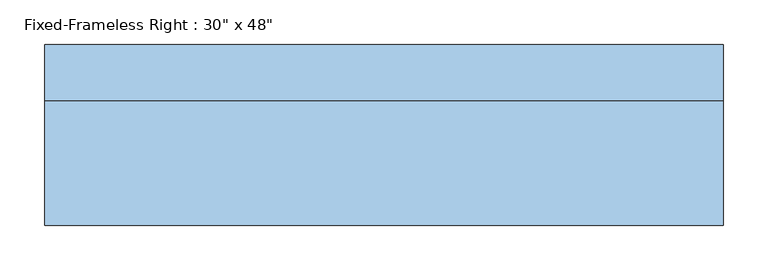
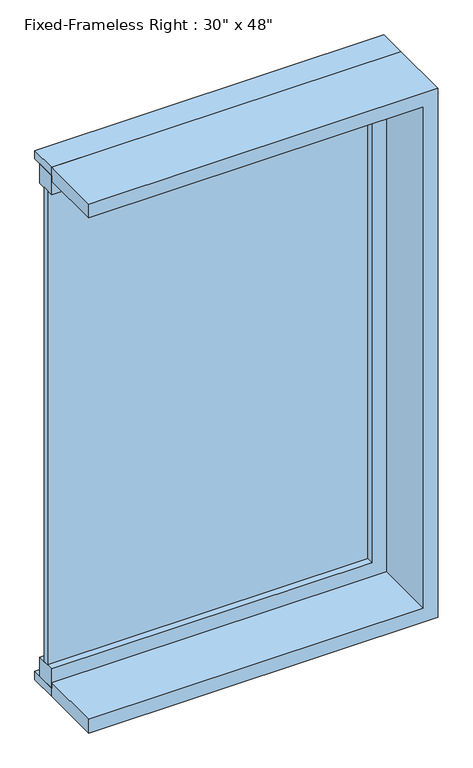
"""IFC4 building model written with IfcOpenShell, lengths in millimetres: window geometry."""

import ifcopenshell
import ifcopenshell.guid

model = None  # the IFC model being written
_history = None  # IfcOwnerHistory: only IFC2X3 demands one
_inside = {}  # id of a spatial element -> (the spatial element, [elements in it])
_under = {}  # id of a project, library or spatial element -> (it, [spatial elements below it])
_declared = {}  # id of a project -> (the project, [libraries it declares])
_typed = {}  # id of a type object -> (the type object, [elements of that type])
_made_of = {}  # id of a material, layer set ... -> (it, [elements and type objects made of it])


def new_model(schema):
    """Start an empty IFC model of exactly this schema.

    Asked for "IFC4X3", IfcOpenShell would pick the latest addendum, in which some entities
    have other attributes; the version numbers below select the first issue.
    IFC2X3 requires an IfcOwnerHistory on every rooted entity: one is made here for all.
    """
    global model, _history
    if schema == "IFC4X3":
        model = ifcopenshell.file(schema_version=(4, 3, 0, 0))
    else:
        model = ifcopenshell.file(schema=schema)
    _inside.clear()
    _under.clear()
    _declared.clear()
    _typed.clear()
    _made_of.clear()
    _history = None
    if model.schema == "IFC2X3":
        org = make("IfcOrganization", Name="unknown")
        user = make(
            "IfcPersonAndOrganization",
            ThePerson=make("IfcPerson", FamilyName="unknown"),
            TheOrganization=org,
        )
        app = make(
            "IfcApplication",
            ApplicationDeveloper=org,
            Version="unknown",
            ApplicationFullName="unknown",
            ApplicationIdentifier="unknown",
        )
        _history = make(
            "IfcOwnerHistory",
            OwningUser=user,
            OwningApplication=app,
            ChangeAction="ADDED",
            CreationDate=0,
        )
    return model


def make(cls, **values):
    """One entity of the class cls with the attributes given. An attribute that is None is left unset."""
    return model.create_entity(
        cls, **{name: value for name, value in values.items() if value is not None}
    )


def rooted(cls, **values):
    """An entity with a GlobalId (a new one), such as an element, a storey or a relation."""
    return make(cls, GlobalId=ifcopenshell.guid.new(), OwnerHistory=_history, **values)


def si_unit(unit_type, name, prefix=None):
    """IfcSIUnit, for example si_unit("LENGTHUNIT", "METRE", prefix="MILLI")."""
    return make("IfcSIUnit", UnitType=unit_type, Prefix=prefix, Name=name)


def assignment(units):
    """IfcUnitAssignment: the units of a project."""
    return None if units is None else make("IfcUnitAssignment", Units=units)


def point(xyz):
    """IfcCartesianPoint."""
    return None if xyz is None else make("IfcCartesianPoint", Coordinates=xyz)


def direction(xyz):
    """IfcDirection."""
    return None if xyz is None else make("IfcDirection", DirectionRatios=xyz)


def frame(location, z_axis=None, x_axis=None):
    """IfcAxis2Placement3D, a coordinate frame: its origin and axes. An axis left out is left unset."""
    return make(
        "IfcAxis2Placement3D",
        Location=point(location),
        Axis=direction(z_axis),
        RefDirection=direction(x_axis),
    )


def origin():
    """The frame at (0, 0, 0) with its axes left unset."""
    return frame((0.0, 0.0, 0.0))


def place(relative_to, where):
    """IfcLocalPlacement: puts the frame where relative to a parent placement (None: the world)."""
    return make(
        "IfcLocalPlacement", PlacementRelTo=relative_to, RelativePlacement=where
    )


def context(
    kind, dimensions, precision=None, world=None, true_north=None, identifier=None
):
    """IfcGeometricRepresentationContext, for example the 3D "Model" context."""
    return make(
        "IfcGeometricRepresentationContext",
        ContextIdentifier=identifier,
        ContextType=kind,
        CoordinateSpaceDimension=dimensions,
        Precision=precision,
        WorldCoordinateSystem=world,
        TrueNorth=true_north,
    )


def project(units=None, contexts=None):
    """IfcProject with its units and contexts."""
    return rooted(
        "IfcProject",
        Name="project",
        RepresentationContexts=contexts,
        UnitsInContext=assignment(units),
    )


def spatial(cls, under=None, at=None, **own):
    """A site, building, storey or space (cls), placed at a placement, below another one or the project."""
    s = rooted(cls, ObjectPlacement=at, **own)
    if under is not None:
        _under.setdefault(under.id(), (under, []))[1].append(s)
    return s


def polyline(points):
    """IfcPolyline through the points."""
    return make("IfcPolyline", Points=[point(p) for p in points])


def outline(outer, holes=None, kind="AREA"):
    """IfcArbitraryClosedProfileDef: a profile drawn as a closed curve; with holes, ...WithVoids."""
    if holes is None:
        return make("IfcArbitraryClosedProfileDef", ProfileType=kind, OuterCurve=outer)
    return make(
        "IfcArbitraryProfileDefWithVoids",
        ProfileType=kind,
        OuterCurve=outer,
        InnerCurves=holes,
    )


def extrude(swept, where, along, depth):
    """IfcExtrudedAreaSolid: the profile swept, set in the frame where, extruded along a direction by depth."""
    return make(
        "IfcExtrudedAreaSolid",
        SweptArea=swept,
        Position=where,
        ExtrudedDirection=direction(along),
        Depth=depth,
    )


def shape(context_of_items, identifier, shape_type, items):
    """IfcShapeRepresentation: the items that make up one representation, for example the "Body"."""
    return make(
        "IfcShapeRepresentation",
        ContextOfItems=context_of_items,
        RepresentationIdentifier=identifier,
        RepresentationType=shape_type,
        Items=items,
    )


def source(mapping_origin, context_of_items, identifier, shape_type, items):
    """IfcRepresentationMap: a shape defined once, which mapped items show again and again."""
    return make(
        "IfcRepresentationMap",
        MappingOrigin=mapping_origin,
        MappedRepresentation=shape(context_of_items, identifier, shape_type, items),
    )


def transform(
    local_origin,
    x_axis=None,
    y_axis=None,
    z_axis=None,
    scale=None,
    scale2=None,
    scale3=None,
    uniform=True,
):
    """IfcCartesianTransformationOperator3D, or its non-uniform kind. x_axis, y_axis, z_axis: its Axis1, 2, 3."""
    if uniform:
        return make(
            "IfcCartesianTransformationOperator3D",
            Axis1=direction(x_axis),
            Axis2=direction(y_axis),
            LocalOrigin=point(local_origin),
            Scale=scale,
            Axis3=direction(z_axis),
        )
    return make(
        "IfcCartesianTransformationOperator3DnonUniform",
        Axis1=direction(x_axis),
        Axis2=direction(y_axis),
        LocalOrigin=point(local_origin),
        Scale=scale,
        Axis3=direction(z_axis),
        Scale2=scale2,
        Scale3=scale3,
    )


def mapped(mapping_source, mapping_target):
    """IfcMappedItem: shows the shape of a source again, moved by a transform."""
    return make(
        "IfcMappedItem", MappingSource=mapping_source, MappingTarget=mapping_target
    )


def made_of(thing, what):
    """Note that an element or type object is made of a material, layer set ...; save() writes the relation."""
    if what is not None:
        _made_of.setdefault(what.id(), (what, []))[1].append(thing)
    return thing


def element(
    cls,
    number,
    at=None,
    inside=None,
    cuts=None,
    type_object=None,
    material=None,
    context=None,
    identifier="Body",
    shape_type=None,
    held_by="IfcProductDefinitionShape",
    body=None,
    shapes=None,
    **own,
):
    """One element of the class cls, such as IfcWall. Its Tag is "e" and its number.

    at: its placement. inside: the storey or other place that contains it. cuts: it is an
    opening in that element (IfcRelVoidsElement). A single representation is given by context,
    identifier, shape_type and body (its items); several are given by shapes. held_by: the class
    of the entity that holds the representations. save() writes the other relations.
    """
    e = rooted(cls, Tag="e%d" % number, ObjectPlacement=at, **own)
    if body is not None:
        shapes = [shape(context, identifier, shape_type, body)]
    if shapes is not None:
        e.Representation = make(held_by, Representations=shapes)
    if inside is not None:
        _inside.setdefault(inside.id(), (inside, []))[1].append(e)
    if cuts is not None:
        rooted(
            "IfcRelVoidsElement", RelatingBuildingElement=cuts, RelatedOpeningElement=e
        )
    if type_object is not None:
        _typed.setdefault(type_object.id(), (type_object, []))[1].append(e)
    return made_of(e, material)


def aggregate(whole, parts):
    """IfcRelAggregates: a whole, such as a stair, and the parts it consists of."""
    return rooted("IfcRelAggregates", RelatingObject=whole, RelatedObjects=parts)


def save(model, path):
    """Write the relations noted so far, then the file.

    IfcRelAggregates (storeys below a building ...), IfcRelContainedInSpatialStructure (elements
    in a storey), IfcRelDefinesByType, IfcRelAssociatesMaterial and IfcRelDeclares: one each for
    every whole, place, type object, material and project.
    """
    for whole, parts in _under.values():
        aggregate(whole, parts)
    for where, things in _inside.values():
        rooted(
            "IfcRelContainedInSpatialStructure",
            RelatedElements=things,
            RelatingStructure=where,
        )
    for kind, things in _typed.values():
        rooted("IfcRelDefinesByType", RelatedObjects=things, RelatingType=kind)
    for what, things in _made_of.values():
        rooted("IfcRelAssociatesMaterial", RelatedObjects=things, RelatingMaterial=what)
    for by, libraries in _declared.values():
        rooted("IfcRelDeclares", RelatingContext=by, RelatedDefinitions=libraries)
    model.write(path)


def window_e8ca31b4(model_context):
    return source(origin(), model_context, "Body", "SweptSolid", [
        extrude(outline(polyline([(279.4, 53.975), (-419.1, 53.975), (-419.1, 66.675), (279.4, 66.675), (279.4, 53.975)])), frame((0.0, 0.0, 977.9), z_axis=(0.0, 0.0, 1.0), x_axis=(1.0, 0.0, 0.0)), (0.0, 0.0, 1.0), 1092.2),
        extrude(outline(polyline([(2114.55, -419.1), (2070.1, -419.1), (2070.1, 279.4), (977.9, 279.4), (977.9, -419.1), (933.45, -419.1), (933.45, 323.85), (2114.55, 323.85), (2114.55, -419.1)])), frame((0.0, 38.1, 0.0), z_axis=(0.0, 1.0, 0.0), x_axis=(0.0, 0.0, 1.0)), (0.0, 0.0, 1.0), 44.45),
        extrude(outline(polyline([(2133.6, -419.1), (2101.85, -419.1), (2101.85, 311.15), (946.15, 311.15), (946.15, -419.1), (914.4, -419.1), (914.4, 342.9), (2133.6, 342.9), (2133.6, -419.1)])), frame((0.0, -101.6, 0.0), z_axis=(0.0, 1.0, 0.0), x_axis=(0.0, 0.0, 1.0)), (0.0, 0.0, 1.0), 139.7),
        extrude(outline(polyline([(2133.6, 342.9), (2133.6, -419.1), (2114.55, -419.1), (2114.55, 323.85), (933.45, 323.85), (933.45, -419.1), (914.4, -419.1), (914.4, 342.9), (2133.6, 342.9)])), frame((0.0, 38.1, 0.0), z_axis=(0.0, 1.0, 0.0), x_axis=(0.0, 0.0, 1.0)), (0.0, 0.0, 1.0), 63.5),
    ])


if __name__ == "__main__":
    model = new_model("IFC4")
    model_context = context("Model", 3, world=origin())
    ifc_project = project(units=[si_unit("LENGTHUNIT", "METRE", prefix="MILLI")], contexts=[model_context])
    site = spatial("IfcSite", under=ifc_project)
    building = spatial("IfcBuilding", under=site)
    placement = place(None, origin())
    window_shape = window_e8ca31b4(model_context)
    element("IfcWindow", 1, ObjectType="Fixed-Frameless Right : 30\" x 48\"", at=placement, inside=building, context=model_context, shape_type="MappedRepresentation", body=[
        mapped(window_shape, transform((0.0, 0.0, 0.0), x_axis=(1.0, 0.0, 0.0), y_axis=(0.0, 1.0, 0.0), z_axis=(0.0, 0.0, 1.0))),
    ])
    save(model, "model.ifc")

# Revit data of these elements
# Type "Fixed-Frameless Right : 30\" x 48\""
#   Type Mark = "76"
#   Assembly Code = "B2020100"
#   Height = 4' - 0"
#   Default Sill Height = 3' - 0"
#   Width = 2' - 6"
#   Window Inset = 0' - 0 3/4"
#   Glass Pane Material = Glass
#   Sash Material = Sash
#   Wall Closure = (empty or 0)
# Element 1 (IfcWindow, "Fixed-Frameless Right : 30\" x 48\"")
#   Materials on its faces: "Sash", "Glass"
# Materials
#   "Glass": class "Glass", colour RGB 0 128 192, transparency 0.75
#   "Sash": class "Wood", colour RGB 224 178 126, transparency 0
